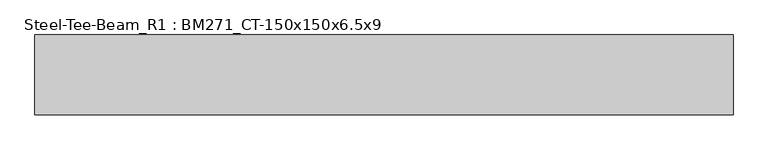
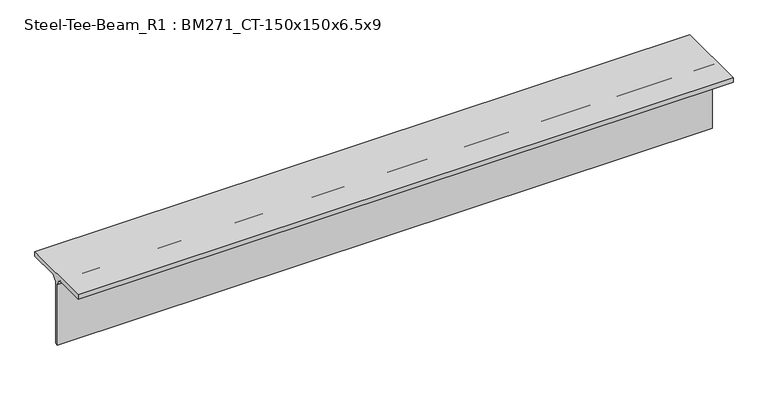
"""IFC4 building model written with IfcOpenShell, lengths in millimetres: member geometry, Steel-Tee-Beam_R1 : BM271_CT-150x150x6.5x9."""

from ifc_helpers import new_model, si_unit, point, frame, frame_2d, origin, place, context, project, spatial, polyline, circle_curve, trimmed, segment, composite_curve, outline, extrude, source, transform, mapped, element, save


def steel_tee_beam_r1_bm271_ct_150x150x6_5x9_6635fbf6(model_context):
    return source(origin(), model_context, "Body", "SweptSolid", [
        extrude(outline(composite_curve([segment(polyline([(75.0, 75.0), (75.0, 66.0), (16.25, 66.0)]), True, "CONTINUOUS"), segment(trimmed(circle_curve(frame_2d((16.25, 53.0)), 13.0), [point((16.25, 66.0))], [point((3.25, 53.0))], True, "CARTESIAN"), True, "CONTINUOUS"), segment(polyline([(3.25, 53.0), (3.25, -75.0), (-3.25, -75.0), (-3.25, 53.0)]), True, "CONTINUOUS"), segment(trimmed(circle_curve(frame_2d((-16.25, 53.0)), 13.0), [point((-3.25, 53.0))], [point((-16.25, 66.0))], True, "CARTESIAN"), True, "CONTINUOUS"), segment(polyline([(-16.25, 66.0), (-75.0, 66.0), (-75.0, 75.0), (75.0, 75.0)]), True, "CONTINUOUS")], self_intersect=False)), frame((-701.7933274, 0.0, 0.0), z_axis=(1.0, 0.0, 0.0), x_axis=(0.0, 1.0, 0.0)), (0.0, 0.0, 1.0), 1311.4188841),
    ])


if __name__ == "__main__":
    model = new_model("IFC4")
    model_context = context("Model", 3, world=origin())
    ifc_project = project(units=[si_unit("LENGTHUNIT", "METRE", prefix="MILLI")], contexts=[model_context])
    site = spatial("IfcSite", under=ifc_project)
    building = spatial("IfcBuilding", under=site)
    placement = place(None, origin())
    steel_tee_beam_r1_bm271_ct_150x150x6_5x9_shape = steel_tee_beam_r1_bm271_ct_150x150x6_5x9_6635fbf6(model_context)
    element("IfcMember", 1, ObjectType="Steel-Tee-Beam_R1 : BM271_CT-150x150x6.5x9", at=placement, inside=building, context=model_context, shape_type="MappedRepresentation", body=[
        mapped(steel_tee_beam_r1_bm271_ct_150x150x6_5x9_shape, transform((0.0, 0.0, 0.0), x_axis=(1.0, 0.0, 0.0), y_axis=(0.0, 1.0, 0.0), z_axis=(0.0, 0.0, 1.0))),
    ])
    save(model, "model.ifc")

# Revit data of these elements
# Type "Steel-Tee-Beam_R1 : BM271_CT-150x150x6.5x9"
#   Keynote = "CT-150x150x6.5x9"
#   Surface Area = 0.588841 m²/m
#   Section Area = 23.3904 cm²
#   Mass per Unit Length = 18.3614 kg/m
#   Length [instance default] = 1.5240 m
#   bf = 0.1500 m
#   d = 0.1500 m
#   k = 0.0220 m
#   r = 0.0130 m
#   tf = 0.0090 m
#   tw = 0.0065 m
#   hec_material4 [instance default] = none
#   hec_material3 [instance default] = none
#   hec_material2 [instance default] = none
#   hec_material1 [instance default] = none
#   Structural Material [instance default] = Steel, 45-345
#   Assembly Code = ""
# Element 1 (IfcMember, "Steel-Tee-Beam_R1 : BM271_CT-150x150x6.5x9")
#   Structural Material = none
# Materials
#   "Steel, 45-345": class "Metal", colour RGB 189 187 185, transparency 0, Description = "Steel 345 MPa", Cost = 0
